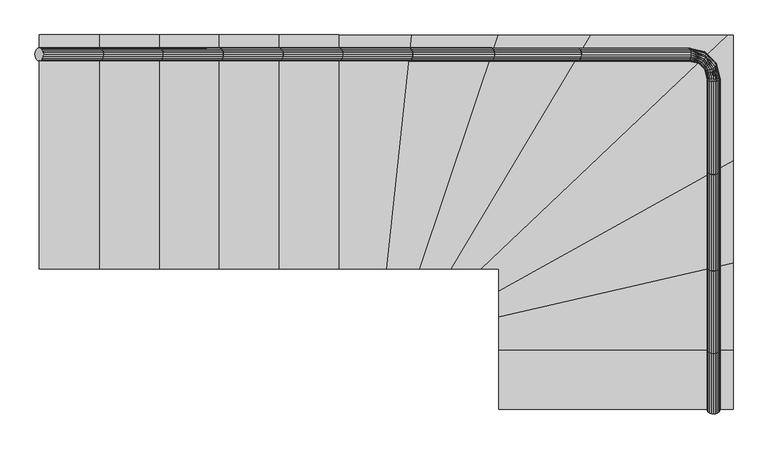
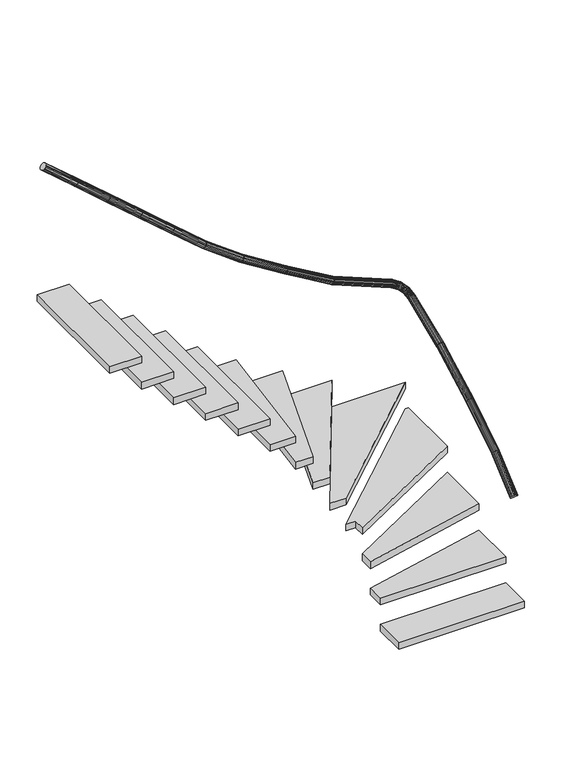
"""IFC4 building model written with IfcOpenShell, lengths in millimetres: stair geometry, 0_3d_modell."""

import ifcopenshell
import ifcopenshell.guid

model = None  # the IFC model being written
_history = None  # IfcOwnerHistory: only IFC2X3 demands one
_inside = {}  # id of a spatial element -> (the spatial element, [elements in it])
_under = {}  # id of a project, library or spatial element -> (it, [spatial elements below it])
_declared = {}  # id of a project -> (the project, [libraries it declares])
_typed = {}  # id of a type object -> (the type object, [elements of that type])
_made_of = {}  # id of a material, layer set ... -> (it, [elements and type objects made of it])


def new_model(schema):
    """Start an empty IFC model of exactly this schema.

    Asked for "IFC4X3", IfcOpenShell would pick the latest addendum, in which some entities
    have other attributes; the version numbers below select the first issue.
    IFC2X3 requires an IfcOwnerHistory on every rooted entity: one is made here for all.
    """
    global model, _history
    if schema == "IFC4X3":
        model = ifcopenshell.file(schema_version=(4, 3, 0, 0))
    else:
        model = ifcopenshell.file(schema=schema)
    _inside.clear()
    _under.clear()
    _declared.clear()
    _typed.clear()
    _made_of.clear()
    _history = None
    if model.schema == "IFC2X3":
        org = make("IfcOrganization", Name="unknown")
        user = make(
            "IfcPersonAndOrganization",
            ThePerson=make("IfcPerson", FamilyName="unknown"),
            TheOrganization=org,
        )
        app = make(
            "IfcApplication",
            ApplicationDeveloper=org,
            Version="unknown",
            ApplicationFullName="unknown",
            ApplicationIdentifier="unknown",
        )
        _history = make(
            "IfcOwnerHistory",
            OwningUser=user,
            OwningApplication=app,
            ChangeAction="ADDED",
            CreationDate=0,
        )
    return model


def make(cls, **values):
    """One entity of the class cls with the attributes given. An attribute that is None is left unset."""
    return model.create_entity(
        cls, **{name: value for name, value in values.items() if value is not None}
    )


def rooted(cls, **values):
    """An entity with a GlobalId (a new one), such as an element, a storey or a relation."""
    return make(cls, GlobalId=ifcopenshell.guid.new(), OwnerHistory=_history, **values)


def si_unit(unit_type, name, prefix=None):
    """IfcSIUnit, for example si_unit("LENGTHUNIT", "METRE", prefix="MILLI")."""
    return make("IfcSIUnit", UnitType=unit_type, Prefix=prefix, Name=name)


def assignment(units):
    """IfcUnitAssignment: the units of a project."""
    return None if units is None else make("IfcUnitAssignment", Units=units)


def point(xyz):
    """IfcCartesianPoint."""
    return None if xyz is None else make("IfcCartesianPoint", Coordinates=xyz)


def direction(xyz):
    """IfcDirection."""
    return None if xyz is None else make("IfcDirection", DirectionRatios=xyz)


def frame(location, z_axis=None, x_axis=None):
    """IfcAxis2Placement3D, a coordinate frame: its origin and axes. An axis left out is left unset."""
    return make(
        "IfcAxis2Placement3D",
        Location=point(location),
        Axis=direction(z_axis),
        RefDirection=direction(x_axis),
    )


def origin():
    """The frame at (0, 0, 0) with its axes left unset."""
    return frame((0.0, 0.0, 0.0))


def origin_with_axes():
    """The frame at (0, 0, 0) with the z axis (0, 0, 1) and the x axis (1, 0, 0) written out."""
    return frame((0.0, 0.0, 0.0), z_axis=(0.0, 0.0, 1.0), x_axis=(1.0, 0.0, 0.0))


def place(relative_to, where):
    """IfcLocalPlacement: puts the frame where relative to a parent placement (None: the world)."""
    return make(
        "IfcLocalPlacement", PlacementRelTo=relative_to, RelativePlacement=where
    )


def context(
    kind, dimensions, precision=None, world=None, true_north=None, identifier=None
):
    """IfcGeometricRepresentationContext, for example the 3D "Model" context."""
    return make(
        "IfcGeometricRepresentationContext",
        ContextIdentifier=identifier,
        ContextType=kind,
        CoordinateSpaceDimension=dimensions,
        Precision=precision,
        WorldCoordinateSystem=world,
        TrueNorth=true_north,
    )


def project(units=None, contexts=None):
    """IfcProject with its units and contexts."""
    return rooted(
        "IfcProject",
        Name="project",
        RepresentationContexts=contexts,
        UnitsInContext=assignment(units),
    )


def spatial(cls, under=None, at=None, **own):
    """A site, building, storey or space (cls), placed at a placement, below another one or the project."""
    s = rooted(cls, ObjectPlacement=at, **own)
    if under is not None:
        _under.setdefault(under.id(), (under, []))[1].append(s)
    return s


def polyline(points):
    """IfcPolyline through the points."""
    return make("IfcPolyline", Points=[point(p) for p in points])


def outline(outer, holes=None, kind="AREA"):
    """IfcArbitraryClosedProfileDef: a profile drawn as a closed curve; with holes, ...WithVoids."""
    if holes is None:
        return make("IfcArbitraryClosedProfileDef", ProfileType=kind, OuterCurve=outer)
    return make(
        "IfcArbitraryProfileDefWithVoids",
        ProfileType=kind,
        OuterCurve=outer,
        InnerCurves=holes,
    )


def extrude(swept, where, along, depth):
    """IfcExtrudedAreaSolid: the profile swept, set in the frame where, extruded along a direction by depth."""
    return make(
        "IfcExtrudedAreaSolid",
        SweptArea=swept,
        Position=where,
        ExtrudedDirection=direction(along),
        Depth=depth,
    )


def faces_of(points, faces, orient=None, outer=None):
    """IfcFace entities. A face is a list of loops; a loop is a list of indices into points, from 0.

    orient and outer hold one flag for each loop. By default every Orientation is true, the
    first loop of a face is its IfcFaceOuterBound and the others are IfcFaceBound.
    """
    made = []
    for i, loops in enumerate(faces):
        bounds = []
        for j, loop in enumerate(loops):
            is_outer = j == 0 if outer is None else outer[i][j]
            bounds.append(
                make(
                    "IfcFaceOuterBound" if is_outer else "IfcFaceBound",
                    Bound=make("IfcPolyLoop", Polygon=[points[k] for k in loop]),
                    Orientation=True if orient is None else orient[i][j],
                )
            )
        made.append(make("IfcFace", Bounds=bounds))
    return made


def faceted_brep(points, faces, orient=None, outer=None, voids=None):
    """IfcFacetedBrep: a solid bounded by flat faces; with voids (closed shells), ...WithVoids."""
    shared = [point(p) for p in points]
    hull = make("IfcClosedShell", CfsFaces=faces_of(shared, faces, orient, outer))
    if voids is None:
        return make("IfcFacetedBrep", Outer=hull)
    return make(
        "IfcFacetedBrepWithVoids",
        Outer=hull,
        Voids=[
            make(cls, CfsFaces=faces_of(shared, fs, o, b)) for cls, fs, o, b in voids
        ],
    )


def shape(context_of_items, identifier, shape_type, items):
    """IfcShapeRepresentation: the items that make up one representation, for example the "Body"."""
    return make(
        "IfcShapeRepresentation",
        ContextOfItems=context_of_items,
        RepresentationIdentifier=identifier,
        RepresentationType=shape_type,
        Items=items,
    )


def source(mapping_origin, context_of_items, identifier, shape_type, items):
    """IfcRepresentationMap: a shape defined once, which mapped items show again and again."""
    return make(
        "IfcRepresentationMap",
        MappingOrigin=mapping_origin,
        MappedRepresentation=shape(context_of_items, identifier, shape_type, items),
    )


def transform(
    local_origin,
    x_axis=None,
    y_axis=None,
    z_axis=None,
    scale=None,
    scale2=None,
    scale3=None,
    uniform=True,
):
    """IfcCartesianTransformationOperator3D, or its non-uniform kind. x_axis, y_axis, z_axis: its Axis1, 2, 3."""
    if uniform:
        return make(
            "IfcCartesianTransformationOperator3D",
            Axis1=direction(x_axis),
            Axis2=direction(y_axis),
            LocalOrigin=point(local_origin),
            Scale=scale,
            Axis3=direction(z_axis),
        )
    return make(
        "IfcCartesianTransformationOperator3DnonUniform",
        Axis1=direction(x_axis),
        Axis2=direction(y_axis),
        LocalOrigin=point(local_origin),
        Scale=scale,
        Axis3=direction(z_axis),
        Scale2=scale2,
        Scale3=scale3,
    )


def mapped(mapping_source, mapping_target):
    """IfcMappedItem: shows the shape of a source again, moved by a transform."""
    return make(
        "IfcMappedItem", MappingSource=mapping_source, MappingTarget=mapping_target
    )


def made_of(thing, what):
    """Note that an element or type object is made of a material, layer set ...; save() writes the relation."""
    if what is not None:
        _made_of.setdefault(what.id(), (what, []))[1].append(thing)
    return thing


def element(
    cls,
    number,
    at=None,
    inside=None,
    cuts=None,
    type_object=None,
    material=None,
    context=None,
    identifier="Body",
    shape_type=None,
    held_by="IfcProductDefinitionShape",
    body=None,
    shapes=None,
    **own,
):
    """One element of the class cls, such as IfcWall. Its Tag is "e" and its number.

    at: its placement. inside: the storey or other place that contains it. cuts: it is an
    opening in that element (IfcRelVoidsElement). A single representation is given by context,
    identifier, shape_type and body (its items); several are given by shapes. held_by: the class
    of the entity that holds the representations. save() writes the other relations.
    """
    e = rooted(cls, Tag="e%d" % number, ObjectPlacement=at, **own)
    if body is not None:
        shapes = [shape(context, identifier, shape_type, body)]
    if shapes is not None:
        e.Representation = make(held_by, Representations=shapes)
    if inside is not None:
        _inside.setdefault(inside.id(), (inside, []))[1].append(e)
    if cuts is not None:
        rooted(
            "IfcRelVoidsElement", RelatingBuildingElement=cuts, RelatedOpeningElement=e
        )
    if type_object is not None:
        _typed.setdefault(type_object.id(), (type_object, []))[1].append(e)
    return made_of(e, material)


def aggregate(whole, parts):
    """IfcRelAggregates: a whole, such as a stair, and the parts it consists of."""
    return rooted("IfcRelAggregates", RelatingObject=whole, RelatedObjects=parts)


def save(model, path):
    """Write the relations noted so far, then the file.

    IfcRelAggregates (storeys below a building ...), IfcRelContainedInSpatialStructure (elements
    in a storey), IfcRelDefinesByType, IfcRelAssociatesMaterial and IfcRelDeclares: one each for
    every whole, place, type object, material and project.
    """
    for whole, parts in _under.values():
        aggregate(whole, parts)
    for where, things in _inside.values():
        rooted(
            "IfcRelContainedInSpatialStructure",
            RelatedElements=things,
            RelatingStructure=where,
        )
    for kind, things in _typed.values():
        rooted("IfcRelDefinesByType", RelatedObjects=things, RelatingType=kind)
    for what, things in _made_of.values():
        rooted("IfcRelAssociatesMaterial", RelatedObjects=things, RelatingMaterial=what)
    for by, libraries in _declared.values():
        rooted("IfcRelDeclares", RelatingContext=by, RelatedDefinitions=libraries)
    model.write(path)


def stair_b834b6f4(model_context):
    return source(origin(), model_context, "Body", "SolidModel", [
        faceted_brep([(1747.6382113, 1405.678272, 2054.1646194), (1751.801684, 1406.9018591, 2060.987808), (1755.9651567, 1405.678272, 2067.8109967), (1759.7210797, 1402.127284, 2073.966284), (1762.701797, 1396.5964904, 2078.8511477), (1764.6155354, 1389.627284, 2081.9874233), (1765.2749647, 1381.9018591, 2083.0681102), (1764.6155354, 1374.1764343, 2081.9874233), (1762.701797, 1367.2072278, 2078.8511477), (1759.7210797, 1361.6764343, 2073.966284), (1755.9651567, 1358.1254462, 2067.8109967), (1751.801684, 1356.9018591, 2060.987808), (1747.6382113, 1358.1254462, 2054.1646194), (1743.8822884, 1361.6764343, 2048.009332), (1740.901571, 1367.2072278, 2043.1244683), (1738.9878327, 1374.1764343, 2039.9881928), (1738.3284034, 1381.9018591, 2038.9075058), (1738.9878327, 1389.627284, 2039.9881928), (1740.901571, 1396.5964904, 2043.1244683), (1743.8822884, 1402.127284, 2048.009332), (1441.1651504, 1405.678272, 2266.1670868), (1436.659926, 1406.9018591, 2259.5592366), (1432.1547015, 1405.678272, 2252.9513864), (1428.0904799, 1402.127284, 2246.9903587), (1424.8650953, 1396.5964904, 2242.2596602), (1422.7942709, 1389.627284, 2239.2223649), (1422.0807134, 1381.9018591, 2238.1757842), (1422.7942709, 1374.1764343, 2239.2223649), (1424.8650953, 1367.2072278, 2242.2596602), (1428.0904799, 1361.6764343, 2246.9903587), (1432.1547015, 1358.1254462, 2252.9513864), (1436.659926, 1356.9018591, 2259.5592366), (1441.1651504, 1358.1254462, 2266.1670868), (1445.2293721, 1361.6764343, 2272.1281145), (1448.4547567, 1367.2072278, 2276.858813), (1450.5255811, 1374.1764343, 2279.8961083), (1451.2391385, 1381.9018591, 2280.942689), (1450.5255811, 1389.627284, 2279.8961083), (1448.4547567, 1396.5964904, 2276.858813), (1445.2293721, 1402.127284, 2272.1281145)], [[[0, 1, 2, 3, 4, 5, 6, 7, 8, 9, 10, 11, 12, 13, 14, 15, 16, 17, 18, 19]], [[20, 21, 22, 23, 24, 25, 26, 27, 28, 29, 30, 31, 32, 33, 34, 35, 36, 37, 38, 39]], [[2, 1, 21, 20]], [[3, 2, 20, 39]], [[4, 3, 39, 38]], [[5, 4, 38, 37]], [[6, 5, 37, 36]], [[7, 6, 36, 35]], [[8, 7, 35, 34]], [[9, 8, 34, 33]], [[10, 9, 33, 32]], [[11, 10, 32, 31]], [[12, 11, 31, 30]], [[13, 12, 30, 29]], [[14, 13, 29, 28]], [[15, 14, 28, 27]], [[16, 15, 27, 26]], [[17, 16, 26, 25]], [[18, 17, 25, 24]], [[19, 18, 24, 23]], [[0, 19, 23, 22]], [[1, 0, 22, 21]]]),
        faceted_brep([(2630.2801086, 566.7337566, 1259.7925307), (2631.5036957, 562.7078511, 1266.7020937), (2630.2801086, 558.6819455, 1273.6116568), (2626.7291206, 555.0501237, 1279.8448636), (2621.198327, 552.1678935, 1284.7915646), (2614.2291206, 550.3173878, 1287.9675421), (2606.5036957, 549.679747, 1289.0619094), (2598.7782709, 550.3173878, 1287.9675421), (2591.8090644, 552.1678935, 1284.7915646), (2586.2782709, 555.0501237, 1279.8448636), (2582.7272828, 558.6819455, 1273.6116568), (2581.5036957, 562.7078511, 1266.7020937), (2582.7272828, 566.7337566, 1259.7925307), (2586.2782709, 570.3655785, 1253.5593239), (2591.8090644, 573.2478087, 1248.6126229), (2598.7782709, 575.0983143, 1245.4366454), (2606.5036957, 575.7359551, 1244.3422781), (2614.2291206, 575.0983143, 1245.4366454), (2621.198327, 573.2478087, 1248.6126229), (2626.7291206, 570.3655785, 1253.5593239), (2630.2801086, 928.1440687, 1472.4992177), (2631.5036957, 931.5827131, 1465.2735223), (2630.2801086, 935.0213576, 1458.0478269), (2626.7291206, 938.1234035, 1451.529433), (2621.198327, 940.5852011, 1446.3564062), (2614.2291206, 942.1657724, 1443.0351186), (2606.5036957, 942.7104002, 1441.8906809), (2598.7782709, 942.1657724, 1443.0351186), (2591.8090644, 940.5852011, 1446.3564062), (2586.2782709, 938.1234035, 1451.529433), (2582.7272828, 935.0213576, 1458.0478269), (2581.5036957, 931.5827131, 1465.2735223), (2582.7272828, 928.1440687, 1472.4992177), (2586.2782709, 925.0420228, 1479.0176117), (2591.8090644, 922.5802252, 1484.1906384), (2598.7782709, 920.9996538, 1487.511926), (2606.5036957, 920.4550261, 1488.6563638), (2614.2291206, 920.9996538, 1487.511926), (2621.198327, 922.5802252, 1484.1906384), (2626.7291206, 925.0420228, 1479.0176117)], [[[0, 1, 2, 3, 4, 5, 6, 7, 8, 9, 10, 11, 12, 13, 14, 15, 16, 17, 18, 19]], [[20, 21, 22, 23, 24, 25, 26, 27, 28, 29, 30, 31, 32, 33, 34, 35, 36, 37, 38, 39]], [[2, 1, 21, 20]], [[3, 2, 20, 39]], [[4, 3, 39, 38]], [[5, 4, 38, 37]], [[6, 5, 37, 36]], [[7, 6, 36, 35]], [[8, 7, 35, 34]], [[9, 8, 34, 33]], [[10, 9, 33, 32]], [[11, 10, 32, 31]], [[12, 11, 31, 30]], [[13, 12, 30, 29]], [[14, 13, 29, 28]], [[15, 14, 28, 27]], [[16, 15, 27, 26]], [[17, 16, 26, 25]], [[18, 17, 25, 24]], [[19, 18, 24, 23]], [[0, 19, 23, 22]], [[1, 0, 22, 21]]]),
        extrude(outline(polyline([(1781.5036957, 246.9018591), (1781.5036957, 373.9346688), (2681.5036957, 579.8690495), (2681.5036957, 246.9018591), (1781.5036957, 246.9018591)])), frame((0.0, 0.0, 198.5714286), z_axis=(0.0, 0.0, 1.0), x_axis=(1.0, 0.0, 0.0)), (0.0, 0.0, 1.0), 50.0),
        extrude(outline(polyline([(706.9018591, 556.9018591), (476.9018591, 556.9018591), (476.9018591, 1456.9018591), (706.9018591, 1456.9018591), (706.9018591, 556.9018591)])), frame((0.0, 0.0, 1985.7142857), z_axis=(0.0, 0.0, 1.0), x_axis=(1.0, 0.0, 0.0)), (0.0, 0.0, 1.0), 50.0),
        extrude(outline(polyline([(1781.5036957, 473.824936), (1781.5036957, 556.9018591), (1711.5036957, 556.9018591), (2658.8332796, 1456.9018591), (2681.5036957, 1456.9018591), (2681.5036957, 973.1970565), (1781.5036957, 473.824936)])), frame((0.0, 0.0, 595.7142857), z_axis=(0.0, 0.0, 1.0), x_axis=(1.0, 0.0, 0.0)), (0.0, 0.0, 1.0), 50.0),
        extrude(outline(polyline([(246.9018591, 556.9018591), (16.9018591, 556.9018591), (16.9018591, 1456.9018591), (246.9018591, 1456.9018591), (246.9018591, 556.9018591)])), frame((0.0, 0.0, 2382.8571429), z_axis=(0.0, 0.0, 1.0), x_axis=(1.0, 0.0, 0.0)), (0.0, 0.0, 1.0), 50.0),
        extrude(outline(polyline([(1.2235871, -7.9923214), (0.0, 0.0), (1.2235871, 7.9923214), (4.7745751, 15.2022987), (10.3053687, 20.9241691), (17.2745751, 24.597836), (25.0, 25.8636953), (32.7254248, 24.597836), (39.6946313, 20.9241691), (45.2254248, 15.2022987), (48.7764129, 7.9923214), (50.0, 0.0), (48.7764129, -7.9923214), (45.2254248, -15.2022986), (39.6946313, -20.9241689), (32.7254248, -24.5978359), (25.0, -25.8636953), (17.2745751, -24.5978359), (10.3053687, -20.9241689), (4.7745751, -15.2022986), (1.2235871, -7.9923214)])), frame((936.9018591, 1406.9018591, 2656.7020937), z_axis=(-0.7569287102857389, 0.0, 0.6534974579485127), x_axis=(0.0, -1.0, 0.0)), (0.0, 0.0, 1.0), 303.8595272),
        extrude(outline(polyline([(1.2235871, -7.9923214), (0.0, 0.0), (1.2235871, 7.9923214), (4.7745751, 15.2022986), (10.3053687, 20.9241691), (17.2745751, 24.5978359), (25.0, 25.8636953), (32.7254248, 24.5978359), (39.6946313, 20.9241691), (45.2254248, 15.2022986), (48.7764129, 7.9923214), (50.0, 0.0), (48.7764129, -7.9923214), (45.2254248, -15.2022986), (39.6946313, -20.9241689), (32.7254248, -24.5978359), (25.0, -25.8636953), (17.2745751, -24.5978359), (10.3053687, -20.9241689), (4.7745751, -15.2022986), (1.2235871, -7.9923214)])), frame((706.9018591, 1406.9018591, 2855.2735223), z_axis=(-0.7569287102857376, 0.0, 0.6534974579485142), x_axis=(0.0, -1.0, 0.0)), (0.0, 0.0, 1.0), 303.8595272),
        faceted_brep([(1161.9138744, 1405.678272, 2451.8781793), (1166.9018591, 1406.9018591, 2458.1306652), (1171.8898438, 1405.678272, 2464.383151), (1176.3895699, 1402.127284, 2470.0236), (1179.9605727, 1396.5964904, 2474.4998856), (1182.2532976, 1389.627284, 2477.3738379), (1183.0433167, 1381.9018591, 2478.3641344), (1182.2532976, 1374.1764343, 2477.3738379), (1179.9605727, 1367.2072278, 2474.4998856), (1176.3895699, 1361.6764343, 2470.0236), (1171.8898438, 1358.1254462, 2464.383151), (1166.9018591, 1356.9018591, 2458.1306652), (1161.9138744, 1358.1254462, 2451.8781793), (1157.4141484, 1361.6764343, 2446.2377304), (1153.8431456, 1367.2072278, 2441.7614447), (1151.5504206, 1374.1764343, 2438.8874925), (1150.7604015, 1381.9018591, 2437.897196), (1151.5504206, 1389.627284, 2438.8874925), (1153.8431456, 1396.5964904, 2441.7614447), (1157.4141484, 1402.127284, 2446.2377304), (942.1248208, 1405.678272, 2662.7517113), (936.9018591, 1406.9018591, 2656.7020937), (931.6788974, 1405.678272, 2650.6524762), (926.9671956, 1402.127284, 2645.1950374), (923.2279679, 1396.5964904, 2640.8639895), (920.8272359, 1389.627284, 2638.0832855), (920.0, 1381.9018591, 2637.1251202), (920.8272359, 1374.1764343, 2638.0832855), (923.2279679, 1367.2072278, 2640.8639895), (926.9671956, 1361.6764343, 2645.1950374), (931.6788974, 1358.1254462, 2650.6524762), (936.9018591, 1356.9018591, 2656.7020937), (942.1248208, 1358.1254462, 2662.7517113), (946.8365226, 1361.6764343, 2668.2091501), (950.5757504, 1367.2072278, 2672.540198), (952.9764824, 1374.1764343, 2675.320902), (953.8037182, 1381.9018591, 2676.2790673), (952.9764824, 1389.627284, 2675.320902), (950.5757504, 1396.5964904, 2672.540198), (946.8365226, 1402.127284, 2668.2091501)], [[[0, 1, 2, 3, 4, 5, 6, 7, 8, 9, 10, 11, 12, 13, 14, 15, 16, 17, 18, 19]], [[20, 21, 22, 23, 24, 25, 26, 27, 28, 29, 30, 31, 32, 33, 34, 35, 36, 37, 38, 39]], [[2, 1, 21, 20]], [[3, 2, 20, 39]], [[4, 3, 39, 38]], [[5, 4, 38, 37]], [[6, 5, 37, 36]], [[7, 6, 36, 35]], [[8, 7, 35, 34]], [[9, 8, 34, 33]], [[10, 9, 33, 32]], [[11, 10, 32, 31]], [[12, 11, 31, 30]], [[13, 12, 30, 29]], [[14, 13, 29, 28]], [[15, 14, 28, 27]], [[16, 15, 27, 26]], [[17, 16, 26, 25]], [[18, 17, 25, 24]], [[19, 18, 24, 23]], [[0, 19, 23, 22]], [[1, 0, 22, 21]]]),
        extrude(outline(polyline([(1.2235871, -7.9923214), (0.0, 0.0), (1.2235871, 7.9923214), (4.7745751, 15.2022986), (10.3053687, 20.924169), (17.2745751, 24.5978359), (25.0, 25.8636953), (32.7254248, 24.5978359), (39.6946313, 20.924169), (45.2254248, 15.2022986), (48.7764129, 7.9923214), (50.0, 0.0), (48.7764129, -7.9923214), (45.2254248, -15.2022986), (39.6946313, -20.924169), (32.7254248, -24.597836), (25.0, -25.8636953), (17.2745751, -24.597836), (10.3053687, -20.924169), (4.7745751, -15.2022986), (1.2235871, -7.9923214)])), frame((246.9018591, 1406.9018591, 3252.4163795), z_axis=(-0.7569287102857456, 0.0, 0.6534974579485049), x_axis=(0.0, -1.0, 0.0)), (0.0, 0.0, 1.0), 303.8595272),
        faceted_brep([(2630.2801086, 935.0213576, 1458.0478269), (2631.5036957, 931.5827131, 1465.2735223), (2630.2801086, 928.1440687, 1472.4992177), (2626.7291206, 925.0420228, 1479.0176117), (2621.198327, 922.5802252, 1484.1906384), (2614.2291206, 920.9996538, 1487.511926), (2606.5036957, 920.4550261, 1488.6563638), (2598.7782709, 920.9996538, 1487.511926), (2591.8090644, 922.5802252, 1484.1906384), (2586.2782709, 925.0420228, 1479.0176117), (2582.7272828, 928.1440687, 1472.4992177), (2581.5036957, 931.5827131, 1465.2735223), (2582.7272828, 935.0213576, 1458.0478269), (2586.2782709, 938.1234035, 1451.529433), (2591.8090644, 940.5852011, 1446.3564062), (2598.7782709, 942.1657724, 1443.0351186), (2606.5036957, 942.7104002, 1441.8906809), (2614.2291206, 942.1657724, 1443.0351186), (2621.198327, 940.5852011, 1446.3564062), (2626.7291206, 938.1234035, 1451.529433), (2630.2801086, 1283.3224302, 1620.3777918), (2631.5036957, 1286.3944101, 1612.9994356), (2630.2801086, 1289.46639, 1605.6210794), (2626.7291206, 1292.2376632, 1598.9649681), (2621.198327, 1294.436958, 1593.6826483), (2614.2291206, 1295.8489921, 1590.2911902), (2606.5036957, 1296.335546, 1589.1225734), (2598.7782709, 1295.8489921, 1590.2911902), (2591.8090644, 1294.436958, 1593.6826483), (2586.2782709, 1292.2376632, 1598.9649681), (2582.7272828, 1289.46639, 1605.6210794), (2581.5036957, 1286.3944101, 1612.9994356), (2582.7272828, 1283.3224302, 1620.3777918), (2586.2782709, 1280.5511571, 1627.0339031), (2591.8090644, 1278.3518623, 1632.3162229), (2598.7782709, 1276.9398281, 1635.707681), (2606.5036957, 1276.4532743, 1636.8762979), (2614.2291206, 1276.9398281, 1635.707681), (2621.198327, 1278.3518623, 1632.3162229), (2626.7291206, 1280.5511571, 1627.0339031)], [[[0, 1, 2, 3, 4, 5, 6, 7, 8, 9, 10, 11, 12, 13, 14, 15, 16, 17, 18, 19]], [[20, 21, 22, 23, 24, 25, 26, 27, 28, 29, 30, 31, 32, 33, 34, 35, 36, 37, 38, 39]], [[2, 1, 21, 20]], [[3, 2, 20, 39]], [[4, 3, 39, 38]], [[5, 4, 38, 37]], [[6, 5, 37, 36]], [[7, 6, 36, 35]], [[8, 7, 35, 34]], [[9, 8, 34, 33]], [[10, 9, 33, 32]], [[11, 10, 32, 31]], [[12, 11, 31, 30]], [[13, 12, 30, 29]], [[14, 13, 29, 28]], [[15, 14, 28, 27]], [[16, 15, 27, 26]], [[17, 16, 26, 25]], [[18, 17, 25, 24]], [[19, 18, 24, 23]], [[0, 19, 23, 22]], [[1, 0, 22, 21]]]),
        extrude(outline(polyline([(1.2235871, -7.9923214), (0.0, 0.0), (1.2235871, 7.9923214), (4.7745751, 15.2022986), (10.3053687, 20.9241691), (17.2745751, 24.5978359), (25.0, 25.8636953), (32.7254248, 24.5978359), (39.6946313, 20.9241691), (45.2254248, 15.2022986), (48.7764129, 7.9923214), (50.0, 0.0), (48.7764129, -7.9923214), (45.2254248, -15.2022986), (39.6946313, -20.924169), (32.7254248, -24.5978359), (25.0, -25.8636953), (17.2745751, -24.5978359), (10.3053687, -20.924169), (4.7745751, -15.2022986), (1.2235871, -7.9923214)])), frame((476.9018591, 1406.9018591, 3053.8449509), z_axis=(-0.7569287102857464, 0.0, 0.6534974579485041), x_axis=(0.0, -1.0, 0.0)), (0.0, 0.0, 1.0), 303.8595272),
        faceted_brep([(2630.2801086, 22.1248208, 863.5096191), (2631.5036957, 16.9018591, 869.5592366), (2630.2801086, 11.6788974, 875.6088541), (2626.7291206, 6.9671956, 881.0662929), (2621.198327, 3.2279679, 885.3973409), (2614.2291206, 0.8272359, 888.1780448), (2606.5036957, 0.0, 889.1362101), (2598.7782709, 0.8272359, 888.1780448), (2591.8090644, 3.2279679, 885.3973409), (2586.2782709, 6.9671956, 881.0662929), (2582.7272828, 11.6788974, 875.6088541), (2581.5036957, 16.9018591, 869.5592366), (2582.7272828, 22.1248208, 863.5096191), (2586.2782709, 26.8365226, 858.0521803), (2591.8090644, 30.5757504, 853.7211323), (2598.7782709, 32.9764824, 850.9404284), (2606.5036957, 33.8037182, 849.9822631), (2614.2291206, 32.9764824, 850.9404284), (2621.198327, 30.5757504, 853.7211323), (2626.7291206, 26.8365226, 858.0521803), (2630.2801086, 242.1361647, 1074.5750662), (2631.5036957, 246.9018591, 1068.1306652), (2630.2801086, 251.6675536, 1061.6862641), (2626.7291206, 255.9667486, 1055.872686), (2621.198327, 259.3786091, 1051.2590042), (2614.2291206, 261.5691584, 1048.2968382), (2606.5036957, 262.3239703, 1047.2761453), (2598.7782709, 261.5691584, 1048.2968382), (2591.8090644, 259.3786091, 1051.2590042), (2586.2782709, 255.9667486, 1055.872686), (2582.7272828, 251.6675536, 1061.6862641), (2581.5036957, 246.9018591, 1068.1306652), (2582.7272828, 242.1361647, 1074.5750662), (2586.2782709, 237.8369696, 1080.3886444), (2591.8090644, 234.4251091, 1085.0023262), (2598.7782709, 232.2345598, 1087.9644922), (2606.5036957, 231.4797479, 1088.985185), (2614.2291206, 232.2345598, 1087.9644922), (2621.198327, 234.4251091, 1085.0023262), (2626.7291206, 237.8369696, 1080.3886444)], [[[0, 1, 2, 3, 4, 5, 6, 7, 8, 9, 10, 11, 12, 13, 14, 15, 16, 17, 18, 19]], [[20, 21, 22, 23, 24, 25, 26, 27, 28, 29, 30, 31, 32, 33, 34, 35, 36, 37, 38, 39]], [[2, 1, 21, 20]], [[3, 2, 20, 39]], [[4, 3, 39, 38]], [[5, 4, 38, 37]], [[6, 5, 37, 36]], [[7, 6, 36, 35]], [[8, 7, 35, 34]], [[9, 8, 34, 33]], [[10, 9, 33, 32]], [[11, 10, 32, 31]], [[12, 11, 31, 30]], [[13, 12, 30, 29]], [[14, 13, 29, 28]], [[15, 14, 28, 27]], [[16, 15, 27, 26]], [[17, 16, 26, 25]], [[18, 17, 25, 24]], [[19, 18, 24, 23]], [[0, 19, 23, 22]], [[1, 0, 22, 21]]]),
        extrude(outline(polyline([(1711.5036957, 556.9018591), (1597.1723093, 556.9018591), (2132.6233472, 1456.9018591), (2658.8332796, 1456.9018591), (1711.5036957, 556.9018591)])), frame((0.0, 0.0, 794.2857143), z_axis=(0.0, 0.0, 1.0), x_axis=(1.0, 0.0, 0.0)), (0.0, 0.0, 1.0), 50.0),
        extrude(outline(polyline([(1781.5036957, 16.9018591), (1781.5036957, 246.9018591), (2681.5036957, 246.9018591), (2681.5036957, 16.9018591), (1781.5036957, 16.9018591)])), origin_with_axes(), (0.0, 0.0, 1.0), 50.0),
        extrude(outline(polyline([(1349.1921789, 556.9018591), (1166.9018591, 556.9018591), (1166.9018591, 1456.9018591), (1444.6115394, 1456.9018591), (1349.1921789, 556.9018591)])), frame((0.0, 0.0, 1390.0), z_axis=(0.0, 0.0, 1.0), x_axis=(1.0, 0.0, 0.0)), (0.0, 0.0, 1.0), 50.0),
        extrude(outline(polyline([(1477.0220692, 556.9018591), (1349.1921789, 556.9018591), (1444.6115394, 1456.9018591), (1776.781649, 1456.9018591), (1477.0220692, 556.9018591)])), frame((0.0, 0.0, 1191.4285714), z_axis=(0.0, 0.0, 1.0), x_axis=(1.0, 0.0, 0.0)), (0.0, 0.0, 1.0), 50.0),
        faceted_brep([(1432.1547015, 1405.678272, 2252.9513864), (1436.659926, 1406.9018591, 2259.5592366), (1441.1651504, 1405.678272, 2266.1670868), (1445.2293721, 1402.127284, 2272.1281145), (1448.4547567, 1396.5964904, 2276.858813), (1450.5255811, 1389.627284, 2279.8961083), (1451.2391385, 1381.9018591, 2280.942689), (1450.5255811, 1374.1764343, 2279.8961083), (1448.4547567, 1367.2072278, 2276.858813), (1445.2293721, 1361.6764343, 2272.1281145), (1441.1651504, 1358.1254462, 2266.1670868), (1436.659926, 1356.9018591, 2259.5592366), (1432.1547015, 1358.1254462, 2252.9513864), (1428.0904799, 1361.6764343, 2246.9903587), (1424.8650953, 1367.2072278, 2242.2596602), (1422.7942709, 1374.1764343, 2239.2223649), (1422.0807134, 1381.9018591, 2238.1757842), (1422.7942709, 1389.627284, 2239.2223649), (1424.8650953, 1396.5964904, 2242.2596602), (1428.0904799, 1402.127284, 2246.9903587), (1171.8898438, 1405.678272, 2464.383151), (1166.9018591, 1406.9018591, 2458.1306652), (1161.9138744, 1405.678272, 2451.8781793), (1157.4141484, 1402.127284, 2446.2377304), (1153.8431456, 1396.5964904, 2441.7614447), (1151.5504206, 1389.627284, 2438.8874925), (1150.7604015, 1381.9018591, 2437.897196), (1151.5504206, 1374.1764343, 2438.8874925), (1153.8431456, 1367.2072278, 2441.7614447), (1157.4141484, 1361.6764343, 2446.2377304), (1161.9138744, 1358.1254462, 2451.8781793), (1166.9018591, 1356.9018591, 2458.1306652), (1171.8898438, 1358.1254462, 2464.383151), (1176.3895699, 1361.6764343, 2470.0236), (1179.9605727, 1367.2072278, 2474.4998856), (1182.2532976, 1374.1764343, 2477.3738379), (1183.0433167, 1381.9018591, 2478.3641344), (1182.2532976, 1389.627284, 2477.3738379), (1179.9605727, 1396.5964904, 2474.4998856), (1176.3895699, 1402.127284, 2470.0236)], [[[0, 1, 2, 3, 4, 5, 6, 7, 8, 9, 10, 11, 12, 13, 14, 15, 16, 17, 18, 19]], [[20, 21, 22, 23, 24, 25, 26, 27, 28, 29, 30, 31, 32, 33, 34, 35, 36, 37, 38, 39]], [[2, 1, 21, 20]], [[3, 2, 20, 39]], [[4, 3, 39, 38]], [[5, 4, 38, 37]], [[6, 5, 37, 36]], [[7, 6, 36, 35]], [[8, 7, 35, 34]], [[9, 8, 34, 33]], [[10, 9, 33, 32]], [[11, 10, 32, 31]], [[12, 11, 31, 30]], [[13, 12, 30, 29]], [[14, 13, 29, 28]], [[15, 14, 28, 27]], [[16, 15, 27, 26]], [[17, 16, 26, 25]], [[18, 17, 25, 24]], [[19, 18, 24, 23]], [[0, 19, 23, 22]], [[1, 0, 22, 21]]]),
        extrude(outline(polyline([(936.9018591, 556.9018591), (706.9018591, 556.9018591), (706.9018591, 1456.9018591), (936.9018591, 1456.9018591), (936.9018591, 556.9018591)])), frame((0.0, 0.0, 1787.1428571), z_axis=(0.0, 0.0, 1.0), x_axis=(1.0, 0.0, 0.0)), (0.0, 0.0, 1.0), 50.0),
        faceted_brep([(2630.2801086, 1289.46639, 1605.6210794), (2631.5036957, 1286.3944101, 1612.9994356), (2630.2801086, 1283.3224302, 1620.3777918), (2626.7291206, 1280.5511571, 1627.0339031), (2621.198327, 1278.3518623, 1632.3162229), (2614.2291206, 1276.9398281, 1635.707681), (2606.5036957, 1276.4532743, 1636.8762979), (2598.7782709, 1276.9398281, 1635.707681), (2591.8090644, 1278.3518623, 1632.3162229), (2586.2782709, 1280.5511571, 1627.0339031), (2582.7272828, 1283.3224302, 1620.3777918), (2581.5036957, 1286.3944101, 1612.9994356), (2582.7272828, 1289.46639, 1605.6210794), (2586.2782709, 1292.2376632, 1598.9649681), (2591.8090644, 1294.436958, 1593.6826483), (2598.7782709, 1295.8489921, 1590.2911902), (2606.5036957, 1296.335546, 1589.1225734), (2614.2291206, 1295.8489921, 1590.2911902), (2621.198327, 1294.436958, 1593.6826483), (2626.7291206, 1292.2376632, 1598.9649681), (2616.4980036, 1348.8501513, 1638.9123688), (2617.3046378, 1344.8271855, 1645.879395), (2615.8855438, 1340.0232633, 1652.1644401), (2612.3796323, 1334.9086261, 1657.1522801), (2607.1300863, 1329.9839302, 1660.3546705), (2600.650768, 1325.7312391, 1661.4581391), (2593.5759183, 1322.5668359, 1660.3546705), (2586.5980727, 1320.8004745, 1657.1522801), (2580.4002713, 1320.6050585, 1652.1644401), (2575.5891981, 1321.9997167, 1645.879395), (2572.6357946, 1324.8479302, 1638.9123688), (2571.8291603, 1328.870896, 1631.9453426), (2573.2482544, 1333.6748181, 1625.6602975), (2576.7541659, 1338.7894554, 1620.6724574), (2582.0037118, 1343.7141513, 1617.470067), (2588.4830301, 1347.9668423, 1616.3665985), (2595.5578799, 1351.1312455, 1617.470067), (2602.5357255, 1352.8976069, 1620.6724574), (2608.7335269, 1353.0930229, 1625.6602975), (2613.5446, 1351.6983647, 1631.9453426), (2573.2894856, 1391.9456089, 1666.2859781), (2576.1190741, 1389.0124344, 1673.2691208), (2577.5017941, 1384.2169558, 1679.5687049), (2577.3022952, 1378.028588, 1684.5680831), (2575.5401057, 1371.0530916, 1687.7778814), (2572.3877211, 1363.9732768, 1688.8839026), (2568.1537188, 1357.4821652, 1687.7778814), (2563.2525523, 1352.215152, 1684.5680831), (2558.163982, 1348.6878091, 1679.5687049), (2553.3861126, 1347.2454175, 1673.2691208), (2549.3866353, 1348.0291684, 1666.2859781), (2546.5570467, 1350.962343, 1659.3028354), (2545.1743267, 1355.7578216, 1653.0032514), (2545.3738257, 1361.9461894, 1648.0038732), (2547.1360151, 1368.9216857, 1644.7940748), (2550.2883997, 1376.0015006, 1643.6880537), (2554.5224021, 1382.4926122, 1644.7940748), (2559.4235686, 1387.7596254, 1648.0038732), (2564.5121389, 1391.2869683, 1653.0032514), (2569.2900082, 1392.7293599, 1659.3028354), (2510.6895066, 1406.9018591, 1691.7803901), (2513.6813624, 1405.678272, 1699.1915978), (2516.3803544, 1402.127284, 1705.8773449), (2518.5222867, 1396.5964904, 1711.1831838), (2519.8974918, 1389.627284, 1714.5897421), (2520.3713552, 1381.9018591, 1715.7635621), (2519.8974918, 1374.1764343, 1714.5897421), (2518.5222867, 1367.2072278, 1711.1831838), (2516.3803544, 1361.6764343, 1705.8773449), (2513.6813624, 1358.1254462, 1699.1915978), (2510.6895066, 1356.9018591, 1691.7803901), (2507.6976509, 1358.1254462, 1684.3691823), (2504.9986588, 1361.6764343, 1677.6834352), (2502.8567266, 1367.2072278, 1672.3775963), (2501.4815215, 1374.1764343, 1668.971038), (2501.0076581, 1381.9018591, 1667.797218), (2501.4815215, 1389.627284, 1668.971038), (2502.8567266, 1396.5964904, 1672.3775963), (2504.9986588, 1402.127284, 1677.6834352), (2507.6976509, 1405.678272, 1684.3691823), (2091.5504886, 1405.678272, 1869.6030507), (2088.0024274, 1406.9018591, 1862.4163795), (2084.4543661, 1405.678272, 1855.2297082), (2081.2536138, 1402.127284, 1848.7465184), (2078.7134824, 1396.5964904, 1843.6014299), (2077.0826177, 1389.627284, 1840.2980797), (2076.52066, 1381.9018591, 1839.1598228), (2077.0826177, 1374.1764343, 1840.2980797), (2078.7134824, 1367.2072278, 1843.6014299), (2081.2536138, 1361.6764343, 1848.7465184), (2084.4543661, 1358.1254462, 1855.2297082), (2088.0024274, 1356.9018591, 1862.4163795), (2091.5504886, 1358.1254462, 1869.6030507), (2094.7512409, 1361.6764343, 1876.0862405), (2097.2913723, 1367.2072278, 1881.231329), (2098.9222371, 1374.1764343, 1884.5346792), (2099.4841948, 1381.9018591, 1885.6729361), (2098.9222371, 1389.627284, 1884.5346792), (2097.2913723, 1396.5964904, 1881.231329), (2094.7512409, 1402.127284, 1876.0862405)], [[[0, 1, 2, 3, 4, 5, 6, 7, 8, 9, 10, 11, 12, 13, 14, 15, 16, 17, 18, 19]], [[2, 1, 20]], [[21, 2, 20]], [[3, 2, 21]], [[22, 3, 21]], [[4, 3, 22]], [[23, 4, 22]], [[5, 4, 23]], [[24, 5, 23]], [[6, 5, 24]], [[25, 6, 24]], [[7, 6, 25]], [[26, 7, 25]], [[8, 7, 26]], [[27, 8, 26]], [[9, 8, 27]], [[28, 9, 27]], [[10, 9, 28]], [[29, 10, 28]], [[11, 10, 29]], [[30, 11, 29]], [[12, 11, 30]], [[31, 12, 30]], [[13, 12, 31]], [[32, 13, 31]], [[14, 13, 32]], [[33, 14, 32]], [[15, 14, 33]], [[34, 15, 33]], [[16, 15, 34]], [[35, 16, 34]], [[17, 16, 35]], [[36, 17, 35]], [[18, 17, 36]], [[37, 18, 36]], [[19, 18, 37]], [[38, 19, 37]], [[0, 19, 38]], [[39, 0, 38]], [[1, 0, 39]], [[20, 1, 39]], [[21, 20, 40]], [[41, 21, 40]], [[22, 21, 41]], [[42, 22, 41]], [[23, 22, 42]], [[43, 23, 42]], [[24, 23, 43]], [[44, 24, 43]], [[25, 24, 44]], [[45, 25, 44]], [[26, 25, 45]], [[46, 26, 45]], [[27, 26, 46]], [[47, 27, 46]], [[28, 27, 47]], [[48, 28, 47]], [[29, 28, 48]], [[49, 29, 48]], [[30, 29, 49]], [[50, 30, 49]], [[31, 30, 50]], [[51, 31, 50]], [[32, 31, 51]], [[52, 32, 51]], [[33, 32, 52]], [[53, 33, 52]], [[34, 33, 53]], [[54, 34, 53]], [[35, 34, 54]], [[55, 35, 54]], [[36, 35, 55]], [[56, 36, 55]], [[37, 36, 56]], [[57, 37, 56]], [[38, 37, 57]], [[58, 38, 57]], [[39, 38, 58]], [[59, 39, 58]], [[20, 39, 59]], [[40, 20, 59]], [[41, 40, 60]], [[61, 41, 60]], [[42, 41, 61]], [[62, 42, 61]], [[43, 42, 62]], [[63, 43, 62]], [[44, 43, 63]], [[64, 44, 63]], [[45, 44, 64]], [[65, 45, 64]], [[46, 45, 65]], [[66, 46, 65]], [[47, 46, 66]], [[67, 47, 66]], [[48, 47, 67]], [[68, 48, 67]], [[49, 48, 68]], [[69, 49, 68]], [[50, 49, 69]], [[70, 50, 69]], [[51, 50, 70]], [[71, 51, 70]], [[52, 51, 71]], [[72, 52, 71]], [[53, 52, 72]], [[73, 53, 72]], [[54, 53, 73]], [[74, 54, 73]], [[55, 54, 74]], [[75, 55, 74]], [[56, 55, 75]], [[76, 56, 75]], [[57, 56, 76]], [[77, 57, 76]], [[58, 57, 77]], [[78, 58, 77]], [[59, 58, 78]], [[79, 59, 78]], [[40, 59, 79]], [[60, 40, 79]], [[80, 81, 82, 83, 84, 85, 86, 87, 88, 89, 90, 91, 92, 93, 94, 95, 96, 97, 98, 99]], [[61, 60, 81, 80]], [[62, 61, 80, 99]], [[63, 62, 99, 98]], [[64, 63, 98, 97]], [[65, 64, 97, 96]], [[66, 65, 96, 95]], [[67, 66, 95, 94]], [[68, 67, 94, 93]], [[69, 68, 93, 92]], [[70, 69, 92, 91]], [[71, 70, 91, 90]], [[72, 71, 90, 89]], [[73, 72, 89, 88]], [[74, 73, 88, 87]], [[75, 74, 87, 86]], [[76, 75, 86, 85]], [[77, 76, 85, 84]], [[78, 77, 84, 83]], [[79, 78, 83, 82]], [[60, 79, 82, 81]]]),
        faceted_brep([(2084.4543661, 1405.678272, 1855.2297082), (2088.0024274, 1406.9018591, 1862.4163795), (2091.5504886, 1405.678272, 1869.6030507), (2094.7512409, 1402.127284, 1876.0862405), (2097.2913723, 1396.5964904, 1881.231329), (2098.9222371, 1389.627284, 1884.5346792), (2099.4841948, 1381.9018591, 1885.6729361), (2098.9222371, 1374.1764343, 1884.5346792), (2097.2913723, 1367.2072278, 1881.231329), (2094.7512409, 1361.6764343, 1876.0862405), (2091.5504886, 1358.1254462, 1869.6030507), (2088.0024274, 1356.9018591, 1862.4163795), (2084.4543661, 1358.1254462, 1855.2297082), (2081.2536138, 1361.6764343, 1848.7465184), (2078.7134824, 1367.2072278, 1843.6014299), (2077.0826177, 1374.1764343, 1840.2980797), (2076.52066, 1381.9018591, 1839.1598228), (2077.0826177, 1389.627284, 1840.2980797), (2078.7134824, 1396.5964904, 1843.6014299), (2081.2536138, 1402.127284, 1848.7465184), (1755.9651567, 1405.678272, 2067.8109967), (1751.801684, 1406.9018591, 2060.987808), (1747.6382113, 1405.678272, 2054.1646194), (1743.8822884, 1402.127284, 2048.009332), (1740.901571, 1396.5964904, 2043.1244683), (1738.9878327, 1389.627284, 2039.9881928), (1738.3284034, 1381.9018591, 2038.9075058), (1738.9878327, 1374.1764343, 2039.9881928), (1740.901571, 1367.2072278, 2043.1244683), (1743.8822884, 1361.6764343, 2048.009332), (1747.6382113, 1358.1254462, 2054.1646194), (1751.801684, 1356.9018591, 2060.987808), (1755.9651567, 1358.1254462, 2067.8109967), (1759.7210797, 1361.6764343, 2073.966284), (1762.701797, 1367.2072278, 2078.8511477), (1764.6155354, 1374.1764343, 2081.9874233), (1765.2749647, 1381.9018591, 2083.0681102), (1764.6155354, 1389.627284, 2081.9874233), (1762.701797, 1396.5964904, 2078.8511477), (1759.7210797, 1402.127284, 2073.966284)], [[[0, 1, 2, 3, 4, 5, 6, 7, 8, 9, 10, 11, 12, 13, 14, 15, 16, 17, 18, 19]], [[20, 21, 22, 23, 24, 25, 26, 27, 28, 29, 30, 31, 32, 33, 34, 35, 36, 37, 38, 39]], [[2, 1, 21, 20]], [[3, 2, 20, 39]], [[4, 3, 39, 38]], [[5, 4, 38, 37]], [[6, 5, 37, 36]], [[7, 6, 36, 35]], [[8, 7, 35, 34]], [[9, 8, 34, 33]], [[10, 9, 33, 32]], [[11, 10, 32, 31]], [[12, 11, 31, 30]], [[13, 12, 30, 29]], [[14, 13, 29, 28]], [[15, 14, 28, 27]], [[16, 15, 27, 26]], [[17, 16, 26, 25]], [[18, 17, 25, 24]], [[19, 18, 24, 23]], [[0, 19, 23, 22]], [[1, 0, 22, 21]]]),
        extrude(outline(polyline([(1781.5036957, 373.9346688), (1781.5036957, 473.824936), (2681.5036957, 973.1970565), (2681.5036957, 579.8690495), (1781.5036957, 373.9346688)])), frame((0.0, 0.0, 397.1428571), z_axis=(0.0, 0.0, 1.0), x_axis=(1.0, 0.0, 0.0)), (0.0, 0.0, 1.0), 50.0),
        faceted_brep([(2630.2801086, 251.6675536, 1061.6862641), (2631.5036957, 246.9018591, 1068.1306652), (2630.2801086, 242.1361647, 1074.5750662), (2626.7291206, 237.8369696, 1080.3886444), (2621.198327, 234.4251091, 1085.0023262), (2614.2291206, 232.2345598, 1087.9644922), (2606.5036957, 231.4797479, 1088.985185), (2598.7782709, 232.2345598, 1087.9644922), (2591.8090644, 234.4251091, 1085.0023262), (2586.2782709, 237.8369696, 1080.3886444), (2582.7272828, 242.1361647, 1074.5750662), (2581.5036957, 246.9018591, 1068.1306652), (2582.7272828, 251.6675536, 1061.6862641), (2586.2782709, 255.9667486, 1055.872686), (2591.8090644, 259.3786091, 1051.2590042), (2598.7782709, 261.5691584, 1048.2968382), (2606.5036957, 262.3239703, 1047.2761453), (2614.2291206, 261.5691584, 1048.2968382), (2621.198327, 259.3786091, 1051.2590042), (2626.7291206, 255.9667486, 1055.872686), (2630.2801086, 558.6819455, 1273.6116568), (2631.5036957, 562.7078511, 1266.7020937), (2630.2801086, 566.7337566, 1259.7925307), (2626.7291206, 570.3655785, 1253.5593239), (2621.198327, 573.2478087, 1248.6126229), (2614.2291206, 575.0983143, 1245.4366454), (2606.5036957, 575.7359551, 1244.3422781), (2598.7782709, 575.0983143, 1245.4366454), (2591.8090644, 573.2478087, 1248.6126229), (2586.2782709, 570.3655785, 1253.5593239), (2582.7272828, 566.7337566, 1259.7925307), (2581.5036957, 562.7078511, 1266.7020937), (2582.7272828, 558.6819455, 1273.6116568), (2586.2782709, 555.0501237, 1279.8448636), (2591.8090644, 552.1678935, 1284.7915646), (2598.7782709, 550.3173878, 1287.9675421), (2606.5036957, 549.679747, 1289.0619094), (2614.2291206, 550.3173878, 1287.9675421), (2621.198327, 552.1678935, 1284.7915646), (2626.7291206, 555.0501237, 1279.8448636)], [[[0, 1, 2, 3, 4, 5, 6, 7, 8, 9, 10, 11, 12, 13, 14, 15, 16, 17, 18, 19]], [[20, 21, 22, 23, 24, 25, 26, 27, 28, 29, 30, 31, 32, 33, 34, 35, 36, 37, 38, 39]], [[2, 1, 21, 20]], [[3, 2, 20, 39]], [[4, 3, 39, 38]], [[5, 4, 38, 37]], [[6, 5, 37, 36]], [[7, 6, 36, 35]], [[8, 7, 35, 34]], [[9, 8, 34, 33]], [[10, 9, 33, 32]], [[11, 10, 32, 31]], [[12, 11, 31, 30]], [[13, 12, 30, 29]], [[14, 13, 29, 28]], [[15, 14, 28, 27]], [[16, 15, 27, 26]], [[17, 16, 26, 25]], [[18, 17, 25, 24]], [[19, 18, 24, 23]], [[0, 19, 23, 22]], [[1, 0, 22, 21]]]),
        extrude(outline(polyline([(476.9018591, 556.9018591), (246.9018591, 556.9018591), (246.9018591, 1456.9018591), (476.9018591, 1456.9018591), (476.9018591, 556.9018591)])), frame((0.0, 0.0, 2184.2857143), z_axis=(0.0, 0.0, 1.0), x_axis=(1.0, 0.0, 0.0)), (0.0, 0.0, 1.0), 50.0),
        extrude(outline(polyline([(1597.1723093, 556.9018591), (1477.0220692, 556.9018591), (1776.781649, 1456.9018591), (2132.6233472, 1456.9018591), (1597.1723093, 556.9018591)])), frame((0.0, 0.0, 992.8571429), z_axis=(0.0, 0.0, 1.0), x_axis=(1.0, 0.0, 0.0)), (0.0, 0.0, 1.0), 50.0),
        extrude(outline(polyline([(1166.9018591, 556.9018591), (936.9018591, 556.9018591), (936.9018591, 1456.9018591), (1166.9018591, 1456.9018591), (1166.9018591, 556.9018591)])), frame((0.0, 0.0, 1588.5714286), z_axis=(0.0, 0.0, 1.0), x_axis=(1.0, 0.0, 0.0)), (0.0, 0.0, 1.0), 50.0),
    ])


if __name__ == "__main__":
    model = new_model("IFC4")
    model_context = context("Model", 3, world=origin())
    ifc_project = project(units=[si_unit("LENGTHUNIT", "METRE", prefix="MILLI")], contexts=[model_context])
    site = spatial("IfcSite", under=ifc_project)
    building = spatial("IfcBuilding", under=site)
    placement = place(None, origin())
    stair_shape = stair_b834b6f4(model_context)
    element("IfcStair", 1, ObjectType="0_3d_modell", at=placement, inside=building, context=model_context, shape_type="MappedRepresentation", body=[
        mapped(stair_shape, transform((0.0, 0.0, 0.0), x_axis=(1.0, 0.0, 0.0), y_axis=(0.0, 1.0, 0.0), z_axis=(0.0, 0.0, 1.0))),
    ])
    save(model, "model.ifc")

# Revit data of these elements
# Element 1 (IfcStair, "0_3d_modell")
#   Materials on its faces: "*1", "weiss"
# Materials
#   "*1": class "Unassigned", colour RGB 175 175 175, transparency 0
#   "weiss": class "Unassigned", colour RGB 255 255 255, transparency 0
